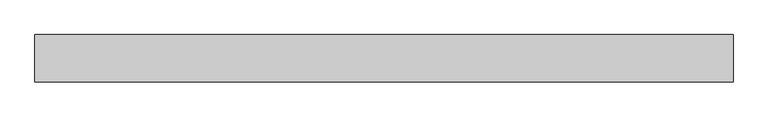
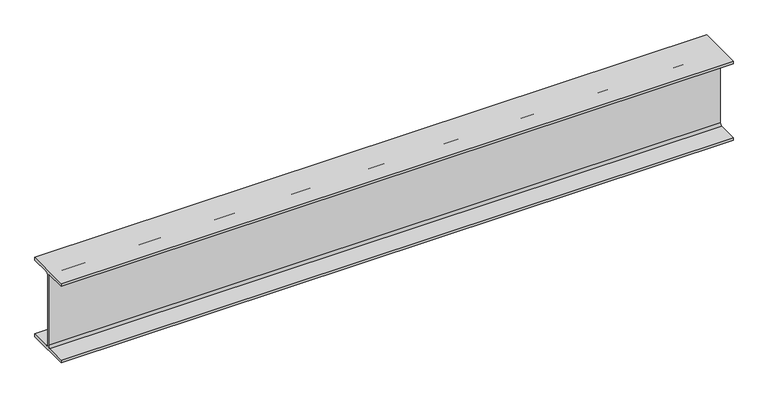
"""IFC4 building model written with IfcOpenShell, lengths in millimetres: beam geometry, Old_Steel Beam_H-KSD3502 : H_SB_ASB_H-194×150x6x9."""

from ifc_helpers import new_model, si_unit, point, frame, frame_2d, origin, place, context, project, spatial, polyline, circle_curve, trimmed, segment, composite_curve, outline, extrude, source, transform, mapped, element, save


def beam_16990a11(model_context):
    return source(origin(), model_context, "Body", "SweptSolid", [
        extrude(outline(composite_curve([segment(polyline([(-82.5, -141.5), (-11.9, -141.5)]), True, "CONTINUOUS"), segment(trimmed(circle_curve(frame_2d((-11.9, -132.6)), 8.9), [point((-11.9, -141.5))], [point((-3.0, -132.6))], True, "CARTESIAN"), True, "CONTINUOUS"), segment(polyline([(-3.0, -132.6), (-3.0, 132.6)]), True, "CONTINUOUS"), segment(trimmed(circle_curve(frame_2d((-11.9, 132.6)), 8.9), [point((-3.0, 132.6))], [point((-11.9, 141.5))], True, "CARTESIAN"), True, "CONTINUOUS"), segment(polyline([(-11.9, 141.5), (-82.5, 141.5), (-82.5, 151.7), (82.5, 151.7), (82.5, 141.5), (11.9, 141.5)]), True, "CONTINUOUS"), segment(trimmed(circle_curve(frame_2d((11.9, 132.6)), 8.9), [point((11.9, 141.5))], [point((3.0, 132.6))], True, "CARTESIAN"), True, "CONTINUOUS"), segment(polyline([(3.0, 132.6), (3.0, -132.6)]), True, "CONTINUOUS"), segment(trimmed(circle_curve(frame_2d((11.9, -132.6)), 8.9), [point((3.0, -132.6))], [point((11.9, -141.5))], True, "CARTESIAN"), True, "CONTINUOUS"), segment(polyline([(11.9, -141.5), (82.5, -141.5), (82.5, -151.7), (-82.5, -151.7), (-82.5, -141.5)]), True, "CONTINUOUS")], self_intersect=False)), frame((-1200.0, 0.0, 0.0), z_axis=(1.0, 0.0, 0.0), x_axis=(0.0, 1.0, 0.0)), (0.0, 0.0, 1.0), 2433.3704936),
    ])


if __name__ == "__main__":
    model = new_model("IFC4")
    model_context = context("Model", 3, world=origin())
    ifc_project = project(units=[si_unit("LENGTHUNIT", "METRE", prefix="MILLI")], contexts=[model_context])
    site = spatial("IfcSite", under=ifc_project)
    building = spatial("IfcBuilding", under=site)
    placement = place(None, origin())
    beam_shape = beam_16990a11(model_context)
    element("IfcBeam", 1, ObjectType="Old_Steel Beam_H-KSD3502 : H_SB_ASB_H-194×150x6x9", at=placement, inside=building, context=model_context, shape_type="MappedRepresentation", body=[
        mapped(beam_shape, transform((0.0, 0.0, 0.0), x_axis=(1.0, 0.0, 0.0), y_axis=(0.0, 1.0, 0.0), z_axis=(0.0, 0.0, 1.0))),
    ])
    save(model, "model.ifc")

# Revit data of these elements
# Type "Old_Steel Beam_H-KSD3502 : H_SB_ASB_H-194×150x6x9"
#   Width = 15.0 cm
#   Web Thickness = 0.6 cm
#   Web Fillet = 1.3 cm
#   Warping Constant = 43316.0 cm⁶
#   Torsional Moment of Inertia = 8.622 cm⁴
#   Torsional Modulus = 1.0 cm³
#   Section Area = 39.01 cm²
#   Plastic Modulus weak axis = 104.0 cm³
#   Plastic Modulus strong axis = 309.0 cm³
#   Perimeter = 0.95 m²/m
#   Nominal Weight = 30.60 kgf/m
#   Moment of Inertia weak axis = 507.00 cm⁴
#   Moment of Inertia strong axis = 2690.00 cm⁴
#   Height = 19.4 cm
#   Flange Thickness = 0.9 cm
#   Elastic Modulus weak axis = 67.6 cm³
#   Elastic Modulus strong axis = 277.0 cm³
#   Centroid Vertical = 9.7 cm
#   Centroid Horizontal = 7.5 cm
#   Length [instance default] = 1.5240 m
#   Structural Material [instance default] = Steel, 45-345
#   Assembly Code = ""
# Element 1 (IfcBeam, "Old_Steel Beam_H-KSD3502 : H_SB_ASB_H-194×150x6x9")
#   Structural Material = none
# Materials
#   "Steel, 45-345": class "Metal", colour RGB 189 187 185, transparency 0, Description = "Steel 345 MPa", Cost = 0
